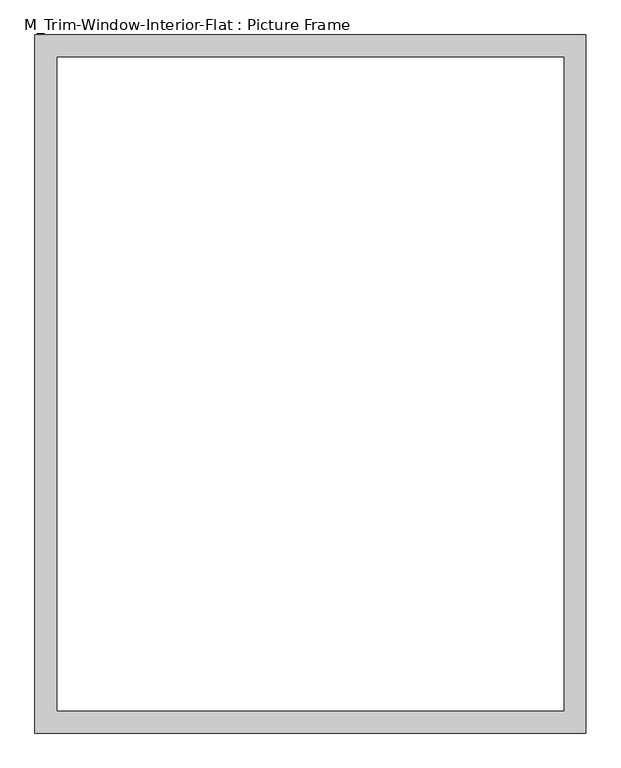
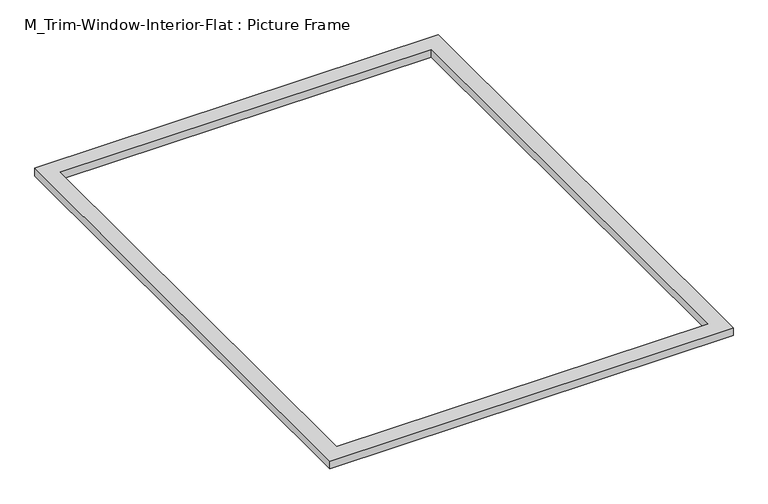
"""IFC4 building model written with IfcOpenShell, lengths in millimetres: proxy geometry, M_Trim-Window-Interior-Flat : Picture Frame."""

import ifcopenshell
import ifcopenshell.guid

model = None  # the IFC model being written
_history = None  # IfcOwnerHistory: only IFC2X3 demands one
_inside = {}  # id of a spatial element -> (the spatial element, [elements in it])
_under = {}  # id of a project, library or spatial element -> (it, [spatial elements below it])
_declared = {}  # id of a project -> (the project, [libraries it declares])
_typed = {}  # id of a type object -> (the type object, [elements of that type])
_made_of = {}  # id of a material, layer set ... -> (it, [elements and type objects made of it])


def new_model(schema):
    """Start an empty IFC model of exactly this schema.

    Asked for "IFC4X3", IfcOpenShell would pick the latest addendum, in which some entities
    have other attributes; the version numbers below select the first issue.
    IFC2X3 requires an IfcOwnerHistory on every rooted entity: one is made here for all.
    """
    global model, _history
    if schema == "IFC4X3":
        model = ifcopenshell.file(schema_version=(4, 3, 0, 0))
    else:
        model = ifcopenshell.file(schema=schema)
    _inside.clear()
    _under.clear()
    _declared.clear()
    _typed.clear()
    _made_of.clear()
    _history = None
    if model.schema == "IFC2X3":
        org = make("IfcOrganization", Name="unknown")
        user = make(
            "IfcPersonAndOrganization",
            ThePerson=make("IfcPerson", FamilyName="unknown"),
            TheOrganization=org,
        )
        app = make(
            "IfcApplication",
            ApplicationDeveloper=org,
            Version="unknown",
            ApplicationFullName="unknown",
            ApplicationIdentifier="unknown",
        )
        _history = make(
            "IfcOwnerHistory",
            OwningUser=user,
            OwningApplication=app,
            ChangeAction="ADDED",
            CreationDate=0,
        )
    return model


def make(cls, **values):
    """One entity of the class cls with the attributes given. An attribute that is None is left unset."""
    return model.create_entity(
        cls, **{name: value for name, value in values.items() if value is not None}
    )


def rooted(cls, **values):
    """An entity with a GlobalId (a new one), such as an element, a storey or a relation."""
    return make(cls, GlobalId=ifcopenshell.guid.new(), OwnerHistory=_history, **values)


def si_unit(unit_type, name, prefix=None):
    """IfcSIUnit, for example si_unit("LENGTHUNIT", "METRE", prefix="MILLI")."""
    return make("IfcSIUnit", UnitType=unit_type, Prefix=prefix, Name=name)


def assignment(units):
    """IfcUnitAssignment: the units of a project."""
    return None if units is None else make("IfcUnitAssignment", Units=units)


def point(xyz):
    """IfcCartesianPoint."""
    return None if xyz is None else make("IfcCartesianPoint", Coordinates=xyz)


def direction(xyz):
    """IfcDirection."""
    return None if xyz is None else make("IfcDirection", DirectionRatios=xyz)


def frame(location, z_axis=None, x_axis=None):
    """IfcAxis2Placement3D, a coordinate frame: its origin and axes. An axis left out is left unset."""
    return make(
        "IfcAxis2Placement3D",
        Location=point(location),
        Axis=direction(z_axis),
        RefDirection=direction(x_axis),
    )


def origin():
    """The frame at (0, 0, 0) with its axes left unset."""
    return frame((0.0, 0.0, 0.0))


def origin_with_axes():
    """The frame at (0, 0, 0) with the z axis (0, 0, 1) and the x axis (1, 0, 0) written out."""
    return frame((0.0, 0.0, 0.0), z_axis=(0.0, 0.0, 1.0), x_axis=(1.0, 0.0, 0.0))


def place(relative_to, where):
    """IfcLocalPlacement: puts the frame where relative to a parent placement (None: the world)."""
    return make(
        "IfcLocalPlacement", PlacementRelTo=relative_to, RelativePlacement=where
    )


def context(
    kind, dimensions, precision=None, world=None, true_north=None, identifier=None
):
    """IfcGeometricRepresentationContext, for example the 3D "Model" context."""
    return make(
        "IfcGeometricRepresentationContext",
        ContextIdentifier=identifier,
        ContextType=kind,
        CoordinateSpaceDimension=dimensions,
        Precision=precision,
        WorldCoordinateSystem=world,
        TrueNorth=true_north,
    )


def project(units=None, contexts=None):
    """IfcProject with its units and contexts."""
    return rooted(
        "IfcProject",
        Name="project",
        RepresentationContexts=contexts,
        UnitsInContext=assignment(units),
    )


def spatial(cls, under=None, at=None, **own):
    """A site, building, storey or space (cls), placed at a placement, below another one or the project."""
    s = rooted(cls, ObjectPlacement=at, **own)
    if under is not None:
        _under.setdefault(under.id(), (under, []))[1].append(s)
    return s


def polyline(points):
    """IfcPolyline through the points."""
    return make("IfcPolyline", Points=[point(p) for p in points])


def outline(outer, holes=None, kind="AREA"):
    """IfcArbitraryClosedProfileDef: a profile drawn as a closed curve; with holes, ...WithVoids."""
    if holes is None:
        return make("IfcArbitraryClosedProfileDef", ProfileType=kind, OuterCurve=outer)
    return make(
        "IfcArbitraryProfileDefWithVoids",
        ProfileType=kind,
        OuterCurve=outer,
        InnerCurves=holes,
    )


def extrude(swept, where, along, depth):
    """IfcExtrudedAreaSolid: the profile swept, set in the frame where, extruded along a direction by depth."""
    return make(
        "IfcExtrudedAreaSolid",
        SweptArea=swept,
        Position=where,
        ExtrudedDirection=direction(along),
        Depth=depth,
    )


def shape(context_of_items, identifier, shape_type, items):
    """IfcShapeRepresentation: the items that make up one representation, for example the "Body"."""
    return make(
        "IfcShapeRepresentation",
        ContextOfItems=context_of_items,
        RepresentationIdentifier=identifier,
        RepresentationType=shape_type,
        Items=items,
    )


def source(mapping_origin, context_of_items, identifier, shape_type, items):
    """IfcRepresentationMap: a shape defined once, which mapped items show again and again."""
    return make(
        "IfcRepresentationMap",
        MappingOrigin=mapping_origin,
        MappedRepresentation=shape(context_of_items, identifier, shape_type, items),
    )


def transform(
    local_origin,
    x_axis=None,
    y_axis=None,
    z_axis=None,
    scale=None,
    scale2=None,
    scale3=None,
    uniform=True,
):
    """IfcCartesianTransformationOperator3D, or its non-uniform kind. x_axis, y_axis, z_axis: its Axis1, 2, 3."""
    if uniform:
        return make(
            "IfcCartesianTransformationOperator3D",
            Axis1=direction(x_axis),
            Axis2=direction(y_axis),
            LocalOrigin=point(local_origin),
            Scale=scale,
            Axis3=direction(z_axis),
        )
    return make(
        "IfcCartesianTransformationOperator3DnonUniform",
        Axis1=direction(x_axis),
        Axis2=direction(y_axis),
        LocalOrigin=point(local_origin),
        Scale=scale,
        Axis3=direction(z_axis),
        Scale2=scale2,
        Scale3=scale3,
    )


def mapped(mapping_source, mapping_target):
    """IfcMappedItem: shows the shape of a source again, moved by a transform."""
    return make(
        "IfcMappedItem", MappingSource=mapping_source, MappingTarget=mapping_target
    )


def made_of(thing, what):
    """Note that an element or type object is made of a material, layer set ...; save() writes the relation."""
    if what is not None:
        _made_of.setdefault(what.id(), (what, []))[1].append(thing)
    return thing


def element(
    cls,
    number,
    at=None,
    inside=None,
    cuts=None,
    type_object=None,
    material=None,
    context=None,
    identifier="Body",
    shape_type=None,
    held_by="IfcProductDefinitionShape",
    body=None,
    shapes=None,
    **own,
):
    """One element of the class cls, such as IfcWall. Its Tag is "e" and its number.

    at: its placement. inside: the storey or other place that contains it. cuts: it is an
    opening in that element (IfcRelVoidsElement). A single representation is given by context,
    identifier, shape_type and body (its items); several are given by shapes. held_by: the class
    of the entity that holds the representations. save() writes the other relations.
    """
    e = rooted(cls, Tag="e%d" % number, ObjectPlacement=at, **own)
    if body is not None:
        shapes = [shape(context, identifier, shape_type, body)]
    if shapes is not None:
        e.Representation = make(held_by, Representations=shapes)
    if inside is not None:
        _inside.setdefault(inside.id(), (inside, []))[1].append(e)
    if cuts is not None:
        rooted(
            "IfcRelVoidsElement", RelatingBuildingElement=cuts, RelatedOpeningElement=e
        )
    if type_object is not None:
        _typed.setdefault(type_object.id(), (type_object, []))[1].append(e)
    return made_of(e, material)


def aggregate(whole, parts):
    """IfcRelAggregates: a whole, such as a stair, and the parts it consists of."""
    return rooted("IfcRelAggregates", RelatingObject=whole, RelatedObjects=parts)


def save(model, path):
    """Write the relations noted so far, then the file.

    IfcRelAggregates (storeys below a building ...), IfcRelContainedInSpatialStructure (elements
    in a storey), IfcRelDefinesByType, IfcRelAssociatesMaterial and IfcRelDeclares: one each for
    every whole, place, type object, material and project.
    """
    for whole, parts in _under.values():
        aggregate(whole, parts)
    for where, things in _inside.values():
        rooted(
            "IfcRelContainedInSpatialStructure",
            RelatedElements=things,
            RelatingStructure=where,
        )
    for kind, things in _typed.values():
        rooted("IfcRelDefinesByType", RelatedObjects=things, RelatingType=kind)
    for what, things in _made_of.values():
        rooted("IfcRelAssociatesMaterial", RelatedObjects=things, RelatingMaterial=what)
    for by, libraries in _declared.values():
        rooted("IfcRelDeclares", RelatingContext=by, RelatedDefinitions=libraries)
    model.write(path)


def m_trim_window_interior_flat_picture_frame_c6c50358(model_context):
    return source(origin(), model_context, "Body", "SweptSolid", [
        extrude(outline(polyline([(747.3, 47.3), (747.3, -1847.3), (-747.3, -1847.3), (-747.3, 47.3), (747.3, 47.3)]), holes=[polyline([(687.3, -12.7), (-687.3, -12.7), (-687.3, -1787.3), (687.3, -1787.3), (687.3, -12.7)])]), origin_with_axes(), (0.0, 0.0, 1.0), 30.0),
    ])


if __name__ == "__main__":
    model = new_model("IFC4")
    model_context = context("Model", 3, world=origin())
    ifc_project = project(units=[si_unit("LENGTHUNIT", "METRE", prefix="MILLI")], contexts=[model_context])
    site = spatial("IfcSite", under=ifc_project)
    building = spatial("IfcBuilding", under=site)
    placement = place(None, origin())
    m_trim_window_interior_flat_picture_frame_shape = m_trim_window_interior_flat_picture_frame_c6c50358(model_context)
    element("IfcBuildingElementProxy", 1, Name="M_Trim-Window-Interior-Flat : Picture Frame", ObjectType="M_Trim-Window-Interior-Flat : Picture Frame", at=placement, inside=building, context=model_context, shape_type="MappedRepresentation", body=[
        mapped(m_trim_window_interior_flat_picture_frame_shape, transform((0.0, 0.0, 0.0), x_axis=(1.0, 0.0, 0.0), y_axis=(0.0, 1.0, 0.0), z_axis=(0.0, 0.0, 1.0))),
    ])
    save(model, "model.ifc")

# Revit data of these elements
# Type "M_Trim-Window-Interior-Flat : Picture Frame"
#   Trim Thickness_Picture Frame = 3 cm
#   Trim Width = 6 cm
#   Trim Thickness_with Sill = 2 cm
#   Sill Thickness = 3 cm
#   Opening Width [instance default] = 60 cm
#   Opening Height [instance default] = 90 cm
#   Default Elevation = 120 cm
#   Sill = no
#   Picture Frame = yes
#   Trim Material [instance default] = none
# Element 1 (IfcBuildingElementProxy, "M_Trim-Window-Interior-Flat : Picture Frame")
#   Opening Width = 140 cm
#   Opening Height = 180 cm
#   Trim Material = Wood - Stained
#   Materials on its faces: "Wood - Stained"
# Materials
#   "Wood - Stained": class "Wood", colour RGB 224 178 126, transparency 0, Cost = 0
